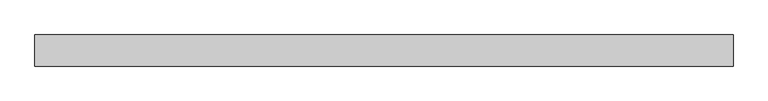
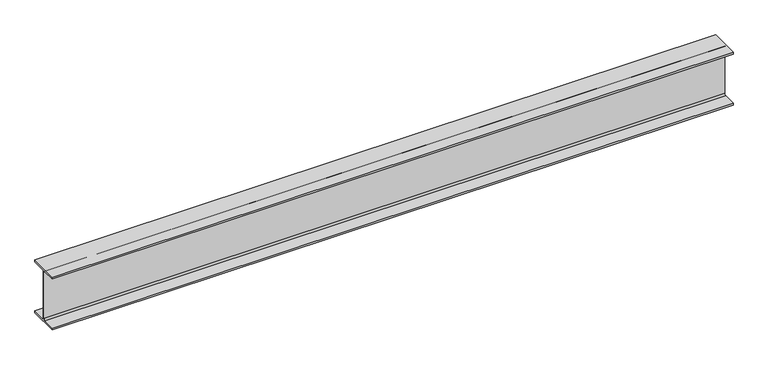
"""IFC4 building model written with IfcOpenShell, lengths in millimetres: beam geometry, Old_Steel Beam_H-KSD3502 : H_SB_ASB_H-200×200x8x12."""

from ifc_helpers import new_model, si_unit, point, frame, frame_2d, origin, place, context, project, spatial, polyline, circle_curve, trimmed, segment, composite_curve, outline, extrude, source, transform, mapped, element, save


def beam_965085ec(model_context):
    return source(origin(), model_context, "Body", "SweptSolid", [
        extrude(outline(composite_curve([segment(polyline([(82.5, -141.5), (82.5, -151.7), (-82.5, -151.7), (-82.5, -141.5), (-11.9, -141.5)]), True, "CONTINUOUS"), segment(trimmed(circle_curve(frame_2d((-11.9, -132.6)), 8.9), [point((-11.9, -141.5))], [point((-3.0, -132.6))], True, "CARTESIAN"), True, "CONTINUOUS"), segment(polyline([(-3.0, -132.6), (-3.0, 132.6)]), True, "CONTINUOUS"), segment(trimmed(circle_curve(frame_2d((-11.9, 132.6)), 8.9), [point((-3.0, 132.6))], [point((-11.9, 141.5))], True, "CARTESIAN"), True, "CONTINUOUS"), segment(polyline([(-11.9, 141.5), (-82.5, 141.5), (-82.5, 151.7), (82.5, 151.7), (82.5, 141.5), (11.9, 141.5)]), True, "CONTINUOUS"), segment(trimmed(circle_curve(frame_2d((11.9, 132.6)), 8.9), [point((11.9, 141.5))], [point((3.0, 132.6))], True, "CARTESIAN"), True, "CONTINUOUS"), segment(polyline([(3.0, 132.6), (3.0, -132.6)]), True, "CONTINUOUS"), segment(trimmed(circle_curve(frame_2d((11.9, -132.6)), 8.9), [point((3.0, -132.6))], [point((11.9, -141.5))], True, "CARTESIAN"), True, "CONTINUOUS"), segment(polyline([(11.9, -141.5), (82.5, -141.5)]), True, "CONTINUOUS")], self_intersect=False)), frame((-1814.9907357, 0.0, 0.0), z_axis=(1.0, 0.0, 0.0), x_axis=(0.0, 1.0, 0.0)), (0.0, 0.0, 1.0), 3702.1907618),
    ])


if __name__ == "__main__":
    model = new_model("IFC4")
    model_context = context("Model", 3, world=origin())
    ifc_project = project(units=[si_unit("LENGTHUNIT", "METRE", prefix="MILLI")], contexts=[model_context])
    site = spatial("IfcSite", under=ifc_project)
    building = spatial("IfcBuilding", under=site)
    placement = place(None, origin())
    beam_shape = beam_965085ec(model_context)
    element("IfcBeam", 1, ObjectType="Old_Steel Beam_H-KSD3502 : H_SB_ASB_H-200×200x8x12", at=placement, inside=building, context=model_context, shape_type="MappedRepresentation", body=[
        mapped(beam_shape, transform((0.0, 0.0, 0.0), x_axis=(1.0, 0.0, 0.0), y_axis=(0.0, 1.0, 0.0), z_axis=(0.0, 0.0, 1.0))),
    ])
    save(model, "model.ifc")

# Revit data of these elements
# Type "Old_Steel Beam_H-KSD3502 : H_SB_ASB_H-200×200x8x12"
#   Width = 20.0 cm
#   Web Thickness = 0.8 cm
#   Web Fillet = 1.3 cm
#   Warping Constant = 141376.0 cm⁶
#   Torsional Moment of Inertia = 26.2485 cm⁴
#   Torsional Modulus = 1.0 cm³
#   Section Area = 63.53 cm²
#   Plastic Modulus weak axis = 244.0 cm³
#   Plastic Modulus strong axis = 525.0 cm³
#   Perimeter = 1.16 m²/m
#   Nominal Weight = 49.90 kgf/m
#   Moment of Inertia weak axis = 1600.00 cm⁴
#   Moment of Inertia strong axis = 4720.00 cm⁴
#   Height = 20.0 cm
#   Flange Thickness = 1.2 cm
#   Elastic Modulus weak axis = 160.0 cm³
#   Elastic Modulus strong axis = 472.0 cm³
#   Centroid Vertical = 10.0 cm
#   Centroid Horizontal = 10.0 cm
#   Length [instance default] = 1.5240 m
#   Structural Material [instance default] = Steel, 45-345
#   Assembly Code = ""
# Element 1 (IfcBeam, "Old_Steel Beam_H-KSD3502 : H_SB_ASB_H-200×200x8x12")
#   Structural Material = none
# Materials
#   "Steel, 45-345": class "Metal", colour RGB 189 187 185, transparency 0, Description = "Steel 345 MPa", Cost = 0
